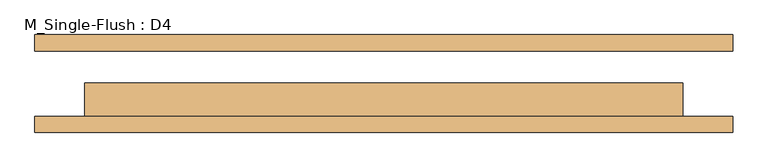
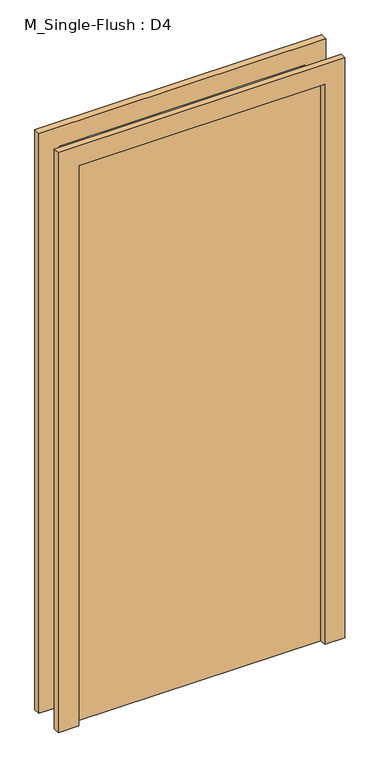
"""IFC4 building model written with IfcOpenShell, lengths in millimetres: door geometry, M_Single-Flush : D4."""

from ifc_helpers import new_model, si_unit, frame, origin, origin_with_axes, place, context, project, spatial, polyline, outline, extrude, source, transform, mapped, element, save


def m_single_flush_d4_5a2dcdb5(model_context):
    return source(origin(), model_context, "Body", "SweptSolid", [
        extrude(outline(polyline([(2286.0, -534.5), (0.0, -534.5), (0.0, -458.5), (2210.0, -458.5), (2210.0, 458.5), (0.0, 458.5), (0.0, 534.5), (2286.0, 534.5), (2286.0, -534.5)])), frame((0.0, -75.0, 0.0), z_axis=(0.0, 1.0, 0.0), x_axis=(0.0, 0.0, 1.0)), (0.0, 0.0, 1.0), 25.0),
        extrude(outline(polyline([(2286.0, 534.5), (2286.0, -534.5), (0.0, -534.5), (0.0, -458.5), (2210.0, -458.5), (2210.0, 458.5), (0.0, 458.5), (0.0, 534.5), (2286.0, 534.5)])), frame((0.0, 50.0, 0.0), z_axis=(0.0, 1.0, 0.0), x_axis=(0.0, 0.0, 1.0)), (0.0, 0.0, 1.0), 25.0),
        extrude(outline(polyline([(458.5, 1.0), (458.5, -50.0), (-458.5, -50.0), (-458.5, 1.0), (458.5, 1.0)])), origin_with_axes(), (0.0, 0.0, 1.0), 2210.0),
    ])


if __name__ == "__main__":
    model = new_model("IFC4")
    model_context = context("Model", 3, world=origin())
    ifc_project = project(units=[si_unit("LENGTHUNIT", "METRE", prefix="MILLI")], contexts=[model_context])
    site = spatial("IfcSite", under=ifc_project)
    building = spatial("IfcBuilding", under=site)
    placement = place(None, origin())
    m_single_flush_d4_shape = m_single_flush_d4_5a2dcdb5(model_context)
    element("IfcDoor", 1, ObjectType="M_Single-Flush : D4", at=placement, inside=building, context=model_context, shape_type="MappedRepresentation", body=[
        mapped(m_single_flush_d4_shape, transform((0.0, 0.0, 0.0), x_axis=(1.0, 0.0, 0.0), y_axis=(0.0, 1.0, 0.0), z_axis=(0.0, 0.0, 1.0))),
    ])
    save(model, "model.ifc")

# Revit data of these elements
# Type "M_Single-Flush : D4"
#   Type Mark = "21"
#   Thickness = 51 mm
#   Height = 2210 mm
#   Trim Projection Ext = 25 mm
#   Trim Projection Int = 25 mm
#   Trim Width = 76 mm
#   Width = 917 mm
#   Door Material = Door - Panel
#   Frame Material = Door - Frame
#   Function = (empty or 0)
#   Wall Closure = (empty or 0)
# Element 1 (IfcDoor, "M_Single-Flush : D4")
#   Materials on its faces: "Door - Frame", "Door - Panel"
# Materials
#   "Door - Panel": class "Wood", colour RGB 210 159 95, transparency 0
#   "Door - Frame": class "Miscellaneous", colour RGB 118 70 51, transparency 0
